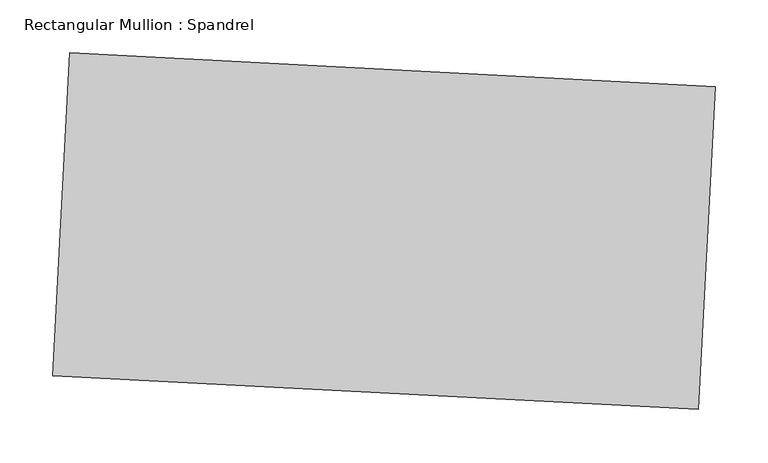
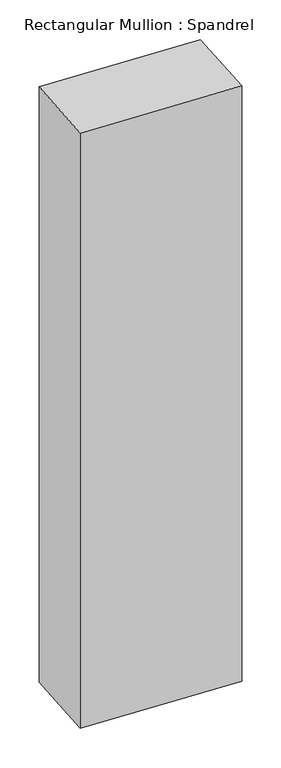
"""IFC4 building model written with IfcOpenShell, lengths in millimetres: member geometry, Rectangular Mullion : Spandrel."""

import ifcopenshell
import ifcopenshell.guid

model = None  # the IFC model being written
_history = None  # IfcOwnerHistory: only IFC2X3 demands one
_inside = {}  # id of a spatial element -> (the spatial element, [elements in it])
_under = {}  # id of a project, library or spatial element -> (it, [spatial elements below it])
_declared = {}  # id of a project -> (the project, [libraries it declares])
_typed = {}  # id of a type object -> (the type object, [elements of that type])
_made_of = {}  # id of a material, layer set ... -> (it, [elements and type objects made of it])


def new_model(schema):
    """Start an empty IFC model of exactly this schema.

    Asked for "IFC4X3", IfcOpenShell would pick the latest addendum, in which some entities
    have other attributes; the version numbers below select the first issue.
    IFC2X3 requires an IfcOwnerHistory on every rooted entity: one is made here for all.
    """
    global model, _history
    if schema == "IFC4X3":
        model = ifcopenshell.file(schema_version=(4, 3, 0, 0))
    else:
        model = ifcopenshell.file(schema=schema)
    _inside.clear()
    _under.clear()
    _declared.clear()
    _typed.clear()
    _made_of.clear()
    _history = None
    if model.schema == "IFC2X3":
        org = make("IfcOrganization", Name="unknown")
        user = make(
            "IfcPersonAndOrganization",
            ThePerson=make("IfcPerson", FamilyName="unknown"),
            TheOrganization=org,
        )
        app = make(
            "IfcApplication",
            ApplicationDeveloper=org,
            Version="unknown",
            ApplicationFullName="unknown",
            ApplicationIdentifier="unknown",
        )
        _history = make(
            "IfcOwnerHistory",
            OwningUser=user,
            OwningApplication=app,
            ChangeAction="ADDED",
            CreationDate=0,
        )
    return model


def make(cls, **values):
    """One entity of the class cls with the attributes given. An attribute that is None is left unset."""
    return model.create_entity(
        cls, **{name: value for name, value in values.items() if value is not None}
    )


def rooted(cls, **values):
    """An entity with a GlobalId (a new one), such as an element, a storey or a relation."""
    return make(cls, GlobalId=ifcopenshell.guid.new(), OwnerHistory=_history, **values)


def si_unit(unit_type, name, prefix=None):
    """IfcSIUnit, for example si_unit("LENGTHUNIT", "METRE", prefix="MILLI")."""
    return make("IfcSIUnit", UnitType=unit_type, Prefix=prefix, Name=name)


def assignment(units):
    """IfcUnitAssignment: the units of a project."""
    return None if units is None else make("IfcUnitAssignment", Units=units)


def point(xyz):
    """IfcCartesianPoint."""
    return None if xyz is None else make("IfcCartesianPoint", Coordinates=xyz)


def direction(xyz):
    """IfcDirection."""
    return None if xyz is None else make("IfcDirection", DirectionRatios=xyz)


def frame(location, z_axis=None, x_axis=None):
    """IfcAxis2Placement3D, a coordinate frame: its origin and axes. An axis left out is left unset."""
    return make(
        "IfcAxis2Placement3D",
        Location=point(location),
        Axis=direction(z_axis),
        RefDirection=direction(x_axis),
    )


def origin():
    """The frame at (0, 0, 0) with its axes left unset."""
    return frame((0.0, 0.0, 0.0))


def place(relative_to, where):
    """IfcLocalPlacement: puts the frame where relative to a parent placement (None: the world)."""
    return make(
        "IfcLocalPlacement", PlacementRelTo=relative_to, RelativePlacement=where
    )


def context(
    kind, dimensions, precision=None, world=None, true_north=None, identifier=None
):
    """IfcGeometricRepresentationContext, for example the 3D "Model" context."""
    return make(
        "IfcGeometricRepresentationContext",
        ContextIdentifier=identifier,
        ContextType=kind,
        CoordinateSpaceDimension=dimensions,
        Precision=precision,
        WorldCoordinateSystem=world,
        TrueNorth=true_north,
    )


def project(units=None, contexts=None):
    """IfcProject with its units and contexts."""
    return rooted(
        "IfcProject",
        Name="project",
        RepresentationContexts=contexts,
        UnitsInContext=assignment(units),
    )


def spatial(cls, under=None, at=None, **own):
    """A site, building, storey or space (cls), placed at a placement, below another one or the project."""
    s = rooted(cls, ObjectPlacement=at, **own)
    if under is not None:
        _under.setdefault(under.id(), (under, []))[1].append(s)
    return s


def polyline(points):
    """IfcPolyline through the points."""
    return make("IfcPolyline", Points=[point(p) for p in points])


def outline(outer, holes=None, kind="AREA"):
    """IfcArbitraryClosedProfileDef: a profile drawn as a closed curve; with holes, ...WithVoids."""
    if holes is None:
        return make("IfcArbitraryClosedProfileDef", ProfileType=kind, OuterCurve=outer)
    return make(
        "IfcArbitraryProfileDefWithVoids",
        ProfileType=kind,
        OuterCurve=outer,
        InnerCurves=holes,
    )


def extrude(swept, where, along, depth):
    """IfcExtrudedAreaSolid: the profile swept, set in the frame where, extruded along a direction by depth."""
    return make(
        "IfcExtrudedAreaSolid",
        SweptArea=swept,
        Position=where,
        ExtrudedDirection=direction(along),
        Depth=depth,
    )


def shape(context_of_items, identifier, shape_type, items):
    """IfcShapeRepresentation: the items that make up one representation, for example the "Body"."""
    return make(
        "IfcShapeRepresentation",
        ContextOfItems=context_of_items,
        RepresentationIdentifier=identifier,
        RepresentationType=shape_type,
        Items=items,
    )


def source(mapping_origin, context_of_items, identifier, shape_type, items):
    """IfcRepresentationMap: a shape defined once, which mapped items show again and again."""
    return make(
        "IfcRepresentationMap",
        MappingOrigin=mapping_origin,
        MappedRepresentation=shape(context_of_items, identifier, shape_type, items),
    )


def transform(
    local_origin,
    x_axis=None,
    y_axis=None,
    z_axis=None,
    scale=None,
    scale2=None,
    scale3=None,
    uniform=True,
):
    """IfcCartesianTransformationOperator3D, or its non-uniform kind. x_axis, y_axis, z_axis: its Axis1, 2, 3."""
    if uniform:
        return make(
            "IfcCartesianTransformationOperator3D",
            Axis1=direction(x_axis),
            Axis2=direction(y_axis),
            LocalOrigin=point(local_origin),
            Scale=scale,
            Axis3=direction(z_axis),
        )
    return make(
        "IfcCartesianTransformationOperator3DnonUniform",
        Axis1=direction(x_axis),
        Axis2=direction(y_axis),
        LocalOrigin=point(local_origin),
        Scale=scale,
        Axis3=direction(z_axis),
        Scale2=scale2,
        Scale3=scale3,
    )


def mapped(mapping_source, mapping_target):
    """IfcMappedItem: shows the shape of a source again, moved by a transform."""
    return make(
        "IfcMappedItem", MappingSource=mapping_source, MappingTarget=mapping_target
    )


def made_of(thing, what):
    """Note that an element or type object is made of a material, layer set ...; save() writes the relation."""
    if what is not None:
        _made_of.setdefault(what.id(), (what, []))[1].append(thing)
    return thing


def element(
    cls,
    number,
    at=None,
    inside=None,
    cuts=None,
    type_object=None,
    material=None,
    context=None,
    identifier="Body",
    shape_type=None,
    held_by="IfcProductDefinitionShape",
    body=None,
    shapes=None,
    **own,
):
    """One element of the class cls, such as IfcWall. Its Tag is "e" and its number.

    at: its placement. inside: the storey or other place that contains it. cuts: it is an
    opening in that element (IfcRelVoidsElement). A single representation is given by context,
    identifier, shape_type and body (its items); several are given by shapes. held_by: the class
    of the entity that holds the representations. save() writes the other relations.
    """
    e = rooted(cls, Tag="e%d" % number, ObjectPlacement=at, **own)
    if body is not None:
        shapes = [shape(context, identifier, shape_type, body)]
    if shapes is not None:
        e.Representation = make(held_by, Representations=shapes)
    if inside is not None:
        _inside.setdefault(inside.id(), (inside, []))[1].append(e)
    if cuts is not None:
        rooted(
            "IfcRelVoidsElement", RelatingBuildingElement=cuts, RelatedOpeningElement=e
        )
    if type_object is not None:
        _typed.setdefault(type_object.id(), (type_object, []))[1].append(e)
    return made_of(e, material)


def aggregate(whole, parts):
    """IfcRelAggregates: a whole, such as a stair, and the parts it consists of."""
    return rooted("IfcRelAggregates", RelatingObject=whole, RelatedObjects=parts)


def save(model, path):
    """Write the relations noted so far, then the file.

    IfcRelAggregates (storeys below a building ...), IfcRelContainedInSpatialStructure (elements
    in a storey), IfcRelDefinesByType, IfcRelAssociatesMaterial and IfcRelDeclares: one each for
    every whole, place, type object, material and project.
    """
    for whole, parts in _under.values():
        aggregate(whole, parts)
    for where, things in _inside.values():
        rooted(
            "IfcRelContainedInSpatialStructure",
            RelatedElements=things,
            RelatingStructure=where,
        )
    for kind, things in _typed.values():
        rooted("IfcRelDefinesByType", RelatedObjects=things, RelatingType=kind)
    for what, things in _made_of.values():
        rooted("IfcRelAssociatesMaterial", RelatedObjects=things, RelatingMaterial=what)
    for by, libraries in _declared.values():
        rooted("IfcRelDeclares", RelatingContext=by, RelatedDefinitions=libraries)
    model.write(path)


def rectangular_mullion_spandrel_10a84132(model_context):
    return source(origin(), model_context, "Body", "SweptSolid", [
        extrude(outline(polyline([(312.3582819, 136.2391416), (296.4062825, -168.1431406), (-312.3582819, -136.2391416), (-296.4062825, 168.1431406), (312.3582819, 136.2391416)])), frame((0.0, 0.0, -2445.9256159), z_axis=(0.0, 0.0, 1.0), x_axis=(1.0, 0.0, 0.0)), (0.0, 0.0, 1.0), 2445.9256159),
    ])


if __name__ == "__main__":
    model = new_model("IFC4")
    model_context = context("Model", 3, world=origin())
    ifc_project = project(units=[si_unit("LENGTHUNIT", "METRE", prefix="MILLI")], contexts=[model_context])
    site = spatial("IfcSite", under=ifc_project)
    building = spatial("IfcBuilding", under=site)
    placement = place(None, origin())
    rectangular_mullion_spandrel_shape = rectangular_mullion_spandrel_10a84132(model_context)
    element("IfcMember", 1, ObjectType="Rectangular Mullion : Spandrel", at=placement, inside=building, context=model_context, shape_type="MappedRepresentation", body=[
        mapped(rectangular_mullion_spandrel_shape, transform((0.0, 0.0, 0.0), x_axis=(1.0, 0.0, 0.0), y_axis=(0.0, 1.0, 0.0), z_axis=(0.0, 0.0, 1.0))),
    ])
    save(model, "model.ifc")

# Revit data of these elements
# Type "Rectangular Mullion : Spandrel"
#   built-in parameter 1007304 = 1 (stored number, unit not read)
#   built-in parameter 1007301 = 1 (stored number, unit not read)
#   built-in parameter 1007300 = 1 (stored number, unit not read)
# Element 1 (IfcMember, "Rectangular Mullion : Spandrel")
#   Materials on its faces: "Aluminum"
# Materials
#   "Aluminum": class "Metal", colour RGB 247 247 247, transparency 0, Description = "Aluminum 6061", Cost = 0
